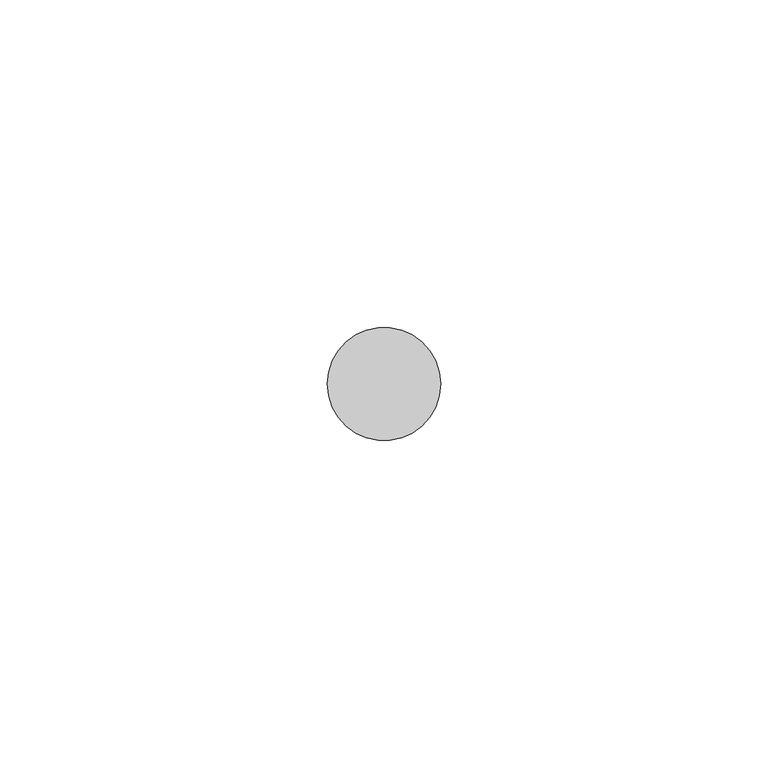
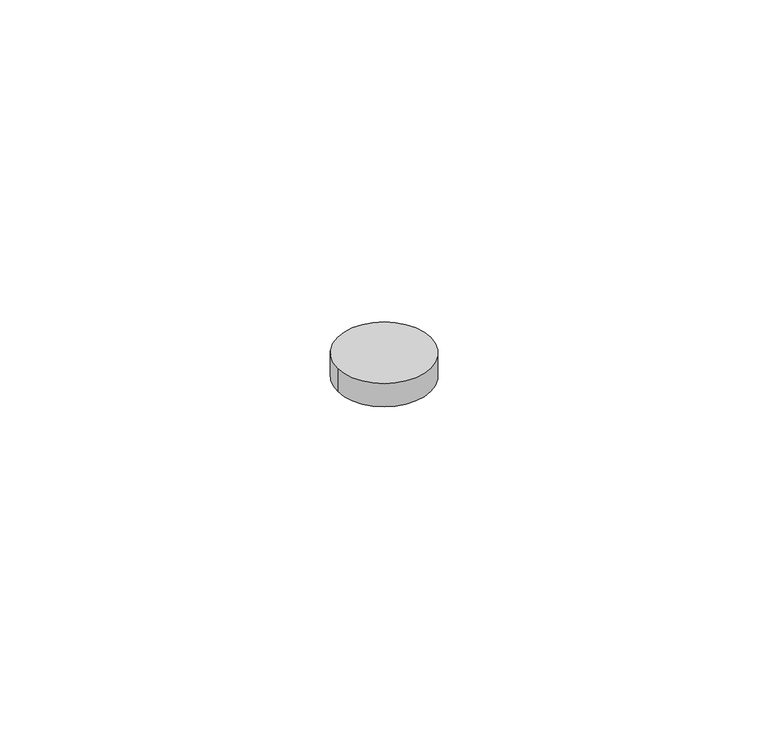
"""IFC4 building model written with IfcOpenShell, lengths in millimetres: proxy geometry, Hinge Pin Keeper10 : Hinge Pin Keeper."""

from ifc_helpers import new_model, si_unit, point, frame, frame_2d, origin, place, context, project, spatial, circle_curve, trimmed, segment, composite_curve, outline, extrude, source, transform, mapped, element, save


def generic_models_3732e641(model_context):
    return source(origin(), model_context, "Body", "SweptSolid", [
        extrude(outline(composite_curve([segment(trimmed(circle_curve(frame_2d((587319.1320739, -536310.3652841)), 8.6534625), [point((587310.4786114, -536310.3652841))], [point((587327.7855364, -536310.3652841))], False, "CARTESIAN"), True, "CONTINUOUS"), segment(trimmed(circle_curve(frame_2d((587319.1320739, -536310.3652841)), 8.6534625), [point((587327.7855364, -536310.3652841))], [point((587310.4786114, -536310.3652841))], False, "CARTESIAN"), True, "CONTINUOUS")], self_intersect=False)), frame((0.0, 0.0, 2084.5859375), z_axis=(0.0, 0.0, 1.0), x_axis=(1.0, 0.0, 0.0)), (0.0, 0.0, 1.0), 4.5640625),
    ])


if __name__ == "__main__":
    model = new_model("IFC4")
    model_context = context("Model", 3, world=origin())
    ifc_project = project(units=[si_unit("LENGTHUNIT", "METRE", prefix="MILLI")], contexts=[model_context])
    site = spatial("IfcSite", under=ifc_project)
    building = spatial("IfcBuilding", under=site)
    placement = place(None, origin())
    generic_models_shape = generic_models_3732e641(model_context)
    element("IfcBuildingElementProxy", 1, Name="Hinge Pin Keeper10 : Hinge Pin Keeper", ObjectType="Hinge Pin Keeper10 : Hinge Pin Keeper", at=placement, inside=building, context=model_context, shape_type="MappedRepresentation", body=[
        mapped(generic_models_shape, transform((0.0, 0.0, 0.0), x_axis=(1.0, 0.0, 0.0), y_axis=(0.0, 1.0, 0.0), z_axis=(0.0, 0.0, 1.0))),
    ])
    save(model, "model.ifc")

# Revit data of these elements
# Element 1 (IfcBuildingElementProxy, "Hinge Pin Keeper10 : Hinge Pin Keeper")
#   Materials on its faces: "6\"X6\" WELD-ON STL BUTT HINGE"
# Materials
#   "6\"X6\" WELD-ON STL BUTT HINGE": class "Metal", colour RGB 189 187 185, transparency 0, Description = "Carbon steel", Cost = 0
